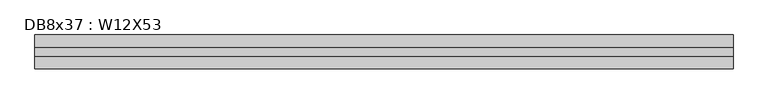
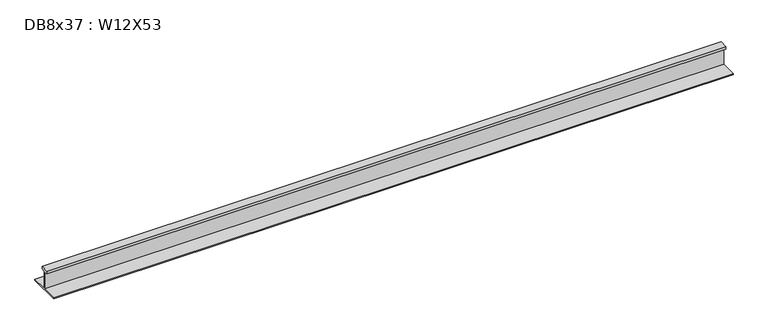
"""IFC4 building model written with IfcOpenShell, lengths in millimetres: beam geometry, DB8x37 : W12X53."""

from ifc_helpers import new_model, si_unit, frame, origin, place, context, project, spatial, polyline, outline, extrude, source, transform, mapped, element, save


def db8x37_w12x53_717e7021(model_context):
    return source(origin(), model_context, "Body", "SweptSolid", [
        extrude(outline(polyline([(38.1, 145.415), (38.1, 120.015), (2.921, 120.015), (2.921, -48.4505), (152.4, -48.4505), (152.4, -58.1025), (-152.4, -58.1025), (-152.4, -48.4505), (-2.921, -48.4505), (-2.921, 120.015), (-38.1, 120.015), (-38.1, 145.415), (38.1, 145.415)])), frame((-3135.63, 0.0, 0.0), z_axis=(1.0, 0.0, 0.0), x_axis=(0.0, 1.0, 0.0)), (0.0, 0.0, 1.0), 6301.359),
    ])


if __name__ == "__main__":
    model = new_model("IFC4")
    model_context = context("Model", 3, world=origin())
    ifc_project = project(units=[si_unit("LENGTHUNIT", "METRE", prefix="MILLI")], contexts=[model_context])
    site = spatial("IfcSite", under=ifc_project)
    building = spatial("IfcBuilding", under=site)
    placement = place(None, origin())
    db8x37_w12x53_shape = db8x37_w12x53_717e7021(model_context)
    element("IfcBeam", 1, ObjectType="DB8x37 : W12X53", at=placement, inside=building, context=model_context, shape_type="MappedRepresentation", body=[
        mapped(db8x37_w12x53_shape, transform((0.0, 0.0, 0.0), x_axis=(1.0, 0.0, 0.0), y_axis=(0.0, 1.0, 0.0), z_axis=(0.0, 0.0, 1.0))),
    ])
    save(model, "model.ifc")

# Revit data of these elements
# Type "DB8x37 : W12X53"
#   Assembly Code = "B10"
#   W = 53
#   Length [instance default] = 5' - 0"
#   bf = 0' - 10"
#   d = 1' - 0.1"
#   k = 0' - 1 3/8"
#   k2 = 0' - 0.8"
#   tf = 0' - 0.575"
#   tw = 0' - 0.345"
#   A = 0.108333 SF
#   Structural Material [instance default] = Steel ASTM A992
# Element 1 (IfcBeam, "DB8x37 : W12X53")
#   Materials on its faces: "Steel ASTM A992"
# Materials
#   "Steel ASTM A992": class "Metal", colour RGB 199 199 199, transparency 0, Description = "Structural steel 50ksi", Cost = 0
